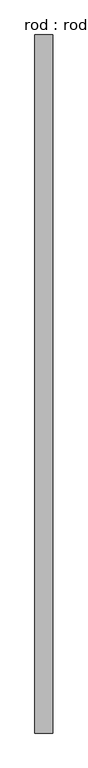
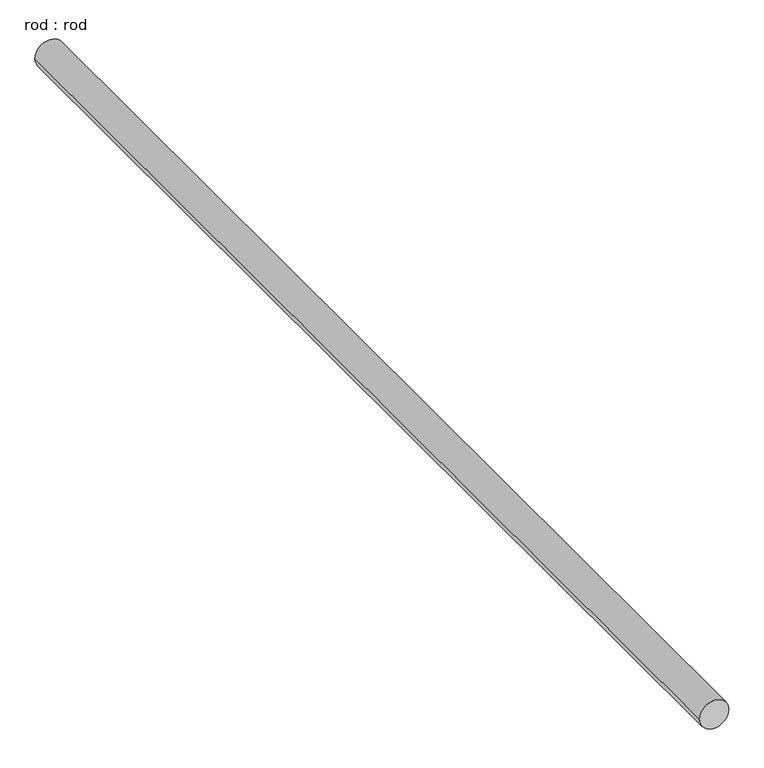
"""IFC4 building model written with IfcOpenShell, lengths in millimetres: proxy geometry, rod : rod."""

from ifc_helpers import new_model, si_unit, point, frame, frame_2d, origin, place, context, project, spatial, circle_curve, trimmed, segment, composite_curve, outline, extrude, source, transform, mapped, element, save


def rod_rod_95c68f3f(model_context):
    return source(origin(), model_context, "Body", "SweptSolid", [
        extrude(outline(composite_curve([segment(trimmed(circle_curve(frame_2d((0.0108462, 0.0)), 200.0), [point((0.0108462, 200.0))], [point((0.0108462, -200.0))], False, "CARTESIAN"), True, "CONTINUOUS"), segment(trimmed(circle_curve(frame_2d((0.0108462, 0.0)), 200.0), [point((0.0108462, -200.0))], [point((0.0108462, 200.0))], False, "CARTESIAN"), True, "CONTINUOUS")], self_intersect=False)), frame((0.0, -3728.6999561, 0.0), z_axis=(0.0, 1.0, 0.0), x_axis=(0.0, 0.0, 1.0)), (0.0, 0.0, 1.0), 15642.8571429),
    ])


if __name__ == "__main__":
    model = new_model("IFC4")
    model_context = context("Model", 3, world=origin())
    ifc_project = project(units=[si_unit("LENGTHUNIT", "METRE", prefix="MILLI")], contexts=[model_context])
    site = spatial("IfcSite", under=ifc_project)
    building = spatial("IfcBuilding", under=site)
    placement = place(None, origin())
    rod_rod_shape = rod_rod_95c68f3f(model_context)
    element("IfcBuildingElementProxy", 1, Name="rod : rod", ObjectType="rod : rod", at=placement, inside=building, context=model_context, shape_type="MappedRepresentation", body=[
        mapped(rod_rod_shape, transform((0.0, 0.0, 0.0), x_axis=(1.0, 0.0, 0.0), y_axis=(0.0, 1.0, 0.0), z_axis=(0.0, 0.0, 1.0))),
    ])
    save(model, "model.ifc")

# Revit data of these elements
# Type "rod : rod"
#   Default Elevation = 0
